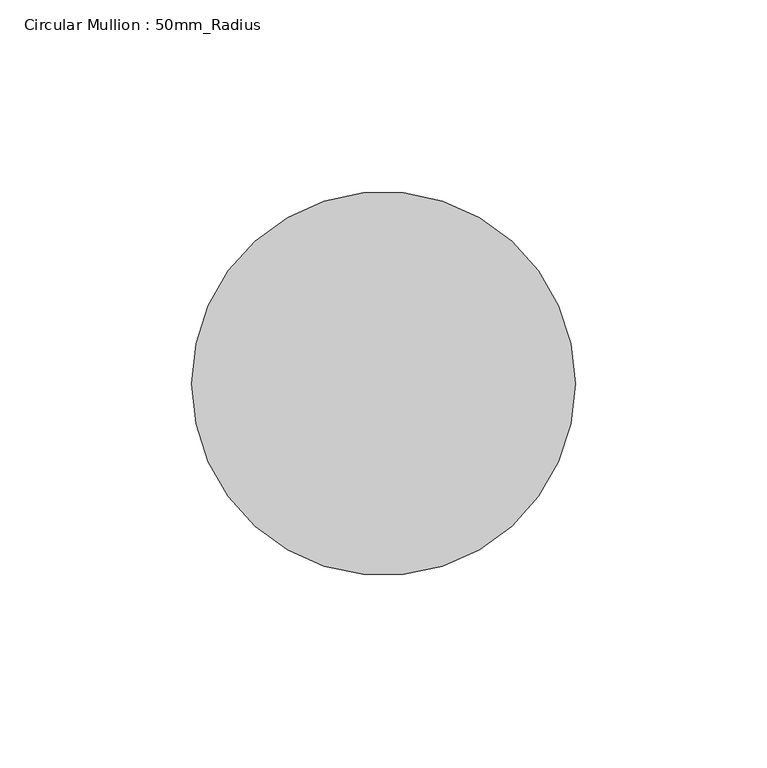
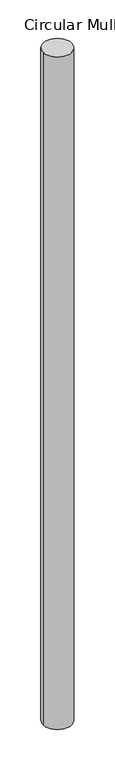
"""IFC4 building model written with IfcOpenShell, lengths in millimetres: member geometry, Circular Mullion : 50mm_Radius."""

from ifc_helpers import new_model, si_unit, point, frame, frame_2d, origin, place, context, project, spatial, circle_curve, trimmed, segment, composite_curve, outline, extrude, source, transform, mapped, element, save


def circular_mullion_50mm_radius_63df8112(model_context):
    return source(origin(), model_context, "Body", "SweptSolid", [
        extrude(outline(composite_curve([segment(trimmed(circle_curve(frame_2d((-50.0, 0.0)), 50.0), [point((0.0, 0.0))], [point((-100.0, 0.0))], False, "CARTESIAN"), True, "CONTINUOUS"), segment(trimmed(circle_curve(frame_2d((-50.0, 0.0)), 50.0), [point((-100.0, 0.0))], [point((0.0, 0.0))], False, "CARTESIAN"), True, "CONTINUOUS")], self_intersect=False)), frame((0.0, 0.0, -2500.0), z_axis=(0.0, 0.0, 1.0), x_axis=(1.0, 0.0, 0.0)), (0.0, 0.0, 1.0), 2500.0),
    ])


if __name__ == "__main__":
    model = new_model("IFC4")
    model_context = context("Model", 3, world=origin())
    ifc_project = project(units=[si_unit("LENGTHUNIT", "METRE", prefix="MILLI")], contexts=[model_context])
    site = spatial("IfcSite", under=ifc_project)
    building = spatial("IfcBuilding", under=site)
    placement = place(None, origin())
    circular_mullion_50mm_radius_shape = circular_mullion_50mm_radius_63df8112(model_context)
    element("IfcMember", 1, ObjectType="Circular Mullion : 50mm_Radius", at=placement, inside=building, context=model_context, shape_type="MappedRepresentation", body=[
        mapped(circular_mullion_50mm_radius_shape, transform((0.0, 0.0, 0.0), x_axis=(1.0, 0.0, 0.0), y_axis=(0.0, 1.0, 0.0), z_axis=(0.0, 0.0, 1.0))),
    ])
    save(model, "model.ifc")

# Revit data of these elements
# Type "Circular Mullion : 50mm_Radius"
#   Keynote = "H11"
#   built-in parameter 1007350 = 0.164042 (stored number, unit not read)
# Element 1 (IfcMember, "Circular Mullion : 50mm_Radius")
#   Materials on its faces: "Aluminium"
# Materials
#   "Aluminium": class "Metal", colour RGB 247 247 247, transparency 0, Description = "Aluminium 6061", Cost = 0
